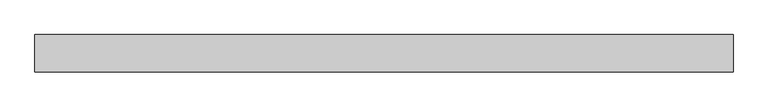
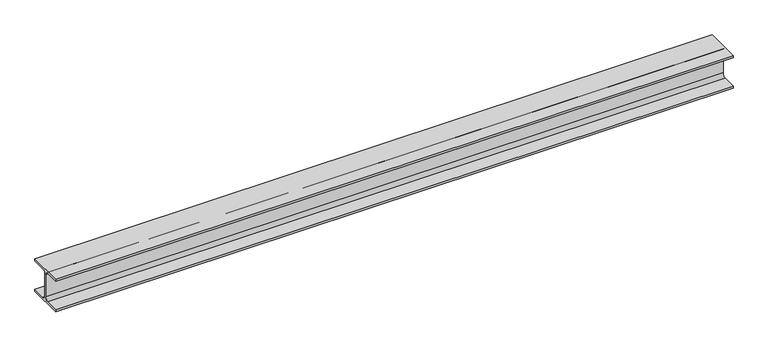
"""IFC4 building model written with IfcOpenShell, lengths in millimetres: beam geometry, NLRS_28_SF_LIB_stalen ligger HEA-AV-CWV-MMBS-SRP_gen_rsf : stalen ligger_gen__HEA 160."""

from ifc_helpers import new_model, si_unit, point, frame, frame_2d, origin, place, context, project, spatial, polyline, circle_curve, trimmed, segment, composite_curve, outline, extrude, source, transform, mapped, element, save


def beam_49e60e2e(model_context):
    return source(origin(), model_context, "Body", "SweptSolid", [
        extrude(outline(composite_curve([segment(polyline([(-80.0, 67.0), (-80.0, 76.0), (80.0, 76.0), (80.0, 67.0), (18.0, 67.0)]), True, "CONTINUOUS"), segment(trimmed(circle_curve(frame_2d((18.0, 52.0)), 15.0), [point((18.0, 67.0))], [point((3.0, 52.0))], True, "CARTESIAN"), True, "CONTINUOUS"), segment(polyline([(3.0, 52.0), (3.0, -52.0)]), True, "CONTINUOUS"), segment(trimmed(circle_curve(frame_2d((18.0, -52.0)), 15.0), [point((3.0, -52.0))], [point((18.0, -67.0))], True, "CARTESIAN"), True, "CONTINUOUS"), segment(polyline([(18.0, -67.0), (80.0, -67.0), (80.0, -76.0), (-80.0, -76.0), (-80.0, -67.0), (-18.0, -67.0)]), True, "CONTINUOUS"), segment(trimmed(circle_curve(frame_2d((-18.0, -52.0)), 15.0), [point((-18.0, -67.0))], [point((-3.0, -52.0))], True, "CARTESIAN"), True, "CONTINUOUS"), segment(polyline([(-3.0, -52.0), (-3.0, 52.0)]), True, "CONTINUOUS"), segment(trimmed(circle_curve(frame_2d((-18.0, 52.0)), 15.0), [point((-3.0, 52.0))], [point((-18.0, 67.0))], True, "CARTESIAN"), True, "CONTINUOUS"), segment(polyline([(-18.0, 67.0), (-80.0, 67.0)]), True, "CONTINUOUS")], self_intersect=False)), frame((-1499.9999994, 0.0, 0.0), z_axis=(1.0, 0.0, 0.0), x_axis=(0.0, 1.0, 0.0)), (0.0, 0.0, 1.0), 2999.9999988),
    ])


if __name__ == "__main__":
    model = new_model("IFC4")
    model_context = context("Model", 3, world=origin())
    ifc_project = project(units=[si_unit("LENGTHUNIT", "METRE", prefix="MILLI")], contexts=[model_context])
    site = spatial("IfcSite", under=ifc_project)
    building = spatial("IfcBuilding", under=site)
    placement = place(None, origin())
    beam_shape = beam_49e60e2e(model_context)
    element("IfcBeam", 1, ObjectType="NLRS_28_SF_LIB_stalen ligger HEA-AV-CWV-MMBS-SRP_gen_rsf : stalen ligger_gen__HEA 160", at=placement, inside=building, context=model_context, shape_type="MappedRepresentation", body=[
        mapped(beam_shape, transform((0.0, 0.0, 0.0), x_axis=(1.0, 0.0, 0.0), y_axis=(0.0, 1.0, 0.0), z_axis=(0.0, 0.0, 1.0))),
    ])
    save(model, "model.ifc")

# Revit data of these elements
# Type "NLRS_28_SF_LIB_stalen ligger HEA-AV-CWV-MMBS-SRP_gen_rsf : stalen ligger_gen__HEA 160"
#   Export Type to IFC As = "IfcBeamType"
#   Type IfcGUID = "3PFmhy1jzBXho9jMrHR46u"
#   Type Comments = "HEA160"
#   Model = " "
#   Manufacturer = " "
#   Fire Rating = " "
#   Description = "stalen ligger HEA160"
#   Assembly Code = "28.11"
#   ra = 15 mm
#   vz = 76 mm
#   vy = 80 mm
#   vpz = 76 mm
#   vpy = 80 mm
#   NLRS_C_lengte [instance default] = 1500 mm
#   Length [instance default] = 1500 mm
#   bf = 160 mm
#   d = 152 mm
#   tf = 9 mm
#   tw = 6 mm
#   Structural Material = NLRS_h2_staal_gen_rsf
#   Keynote = ""
# Element 1 (IfcBeam, "NLRS_28_SF_LIB_stalen ligger HEA-AV-CWV-MMBS-SRP_gen_rsf : stalen ligger_gen__HEA 160")
#   NLRS_C_lengte = 3000 mm
#   Materials on its faces: "NLRS_h2_staal_gen_rsf"
# Materials
#   "NLRS_h2_staal_gen_rsf": class "H - Metaal", colour RGB 189 187 185, transparency 0, Keynote = "h2", Manufacturer = "Revit Standards Foundation", URL = "www.revitstandards.org", Description = "staal", Cost = 0
